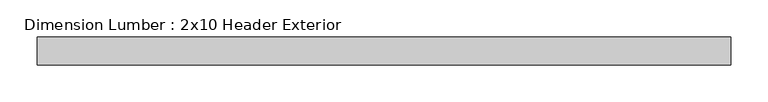
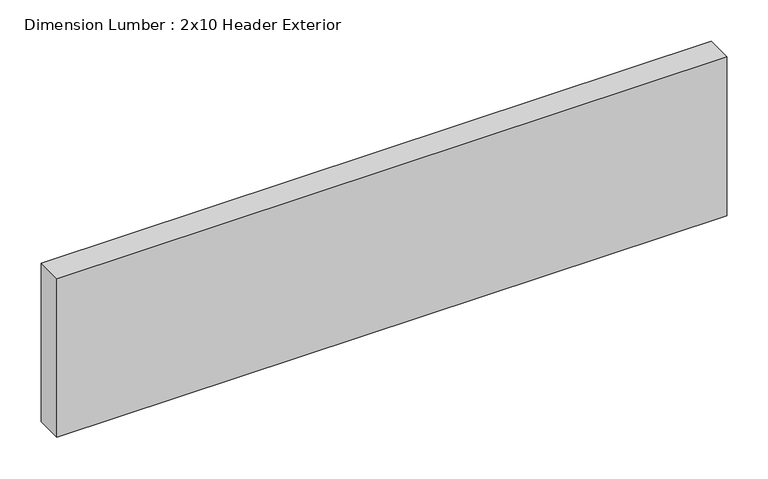
"""IFC4 building model written with IfcOpenShell, lengths in millimetres: beam geometry, Dimension Lumber : 2x10 Header Exterior."""

from ifc_helpers import new_model, si_unit, frame, origin, place, context, project, spatial, polyline, outline, extrude, source, transform, mapped, element, save


def dimension_lumber_2x10_header_exterior_dd7e88d1(model_context):
    return source(origin(), model_context, "Body", "SweptSolid", [
        extrude(outline(polyline([(468.709375, 19.05), (468.709375, -19.05), (-468.709375, -19.05), (-468.709375, 19.05), (468.709375, 19.05)])), frame((0.0, 0.0, -117.475), z_axis=(0.0, 0.0, 1.0), x_axis=(1.0, 0.0, 0.0)), (0.0, 0.0, 1.0), 234.95),
    ])


if __name__ == "__main__":
    model = new_model("IFC4")
    model_context = context("Model", 3, world=origin())
    ifc_project = project(units=[si_unit("LENGTHUNIT", "METRE", prefix="MILLI")], contexts=[model_context])
    site = spatial("IfcSite", under=ifc_project)
    building = spatial("IfcBuilding", under=site)
    placement = place(None, origin())
    dimension_lumber_2x10_header_exterior_shape = dimension_lumber_2x10_header_exterior_dd7e88d1(model_context)
    element("IfcBeam", 1, ObjectType="Dimension Lumber : 2x10 Header Exterior", at=placement, inside=building, context=model_context, shape_type="MappedRepresentation", body=[
        mapped(dimension_lumber_2x10_header_exterior_shape, transform((0.0, 0.0, 0.0), x_axis=(1.0, 0.0, 0.0), y_axis=(0.0, 1.0, 0.0), z_axis=(0.0, 0.0, 1.0))),
    ])
    save(model, "model.ifc")

# Revit data of these elements
# Type "Dimension Lumber : 2x10 Header Exterior"
#   Assembly Code = "B10"
#   A = 0.0963889 SF
#   Length [instance default] = 5' - 0"
#   b = 0' - 1 1/2"
#   d = 0' - 9 1/4"
#   Structural Material [instance default] = Softwood, Lumber
# Element 1 (IfcBeam, "Dimension Lumber : 2x10 Header Exterior")
#   Structural Material = Douglas Fir #2
#   Materials on its faces: "Douglas Fir #2"
# Materials
#   "Softwood, Lumber": class "Wood", colour RGB 223 192 134, transparency 0, Description = "Pinus Echinata", Cost = 0
#   "Douglas Fir #2": class "Wood", colour RGB 223 192 134, transparency 0, Description = "Pinus Echinata", Cost = 0
